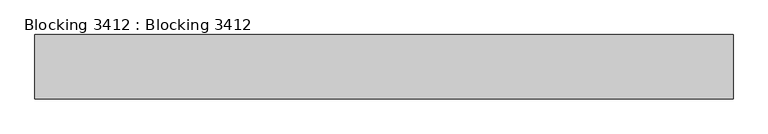
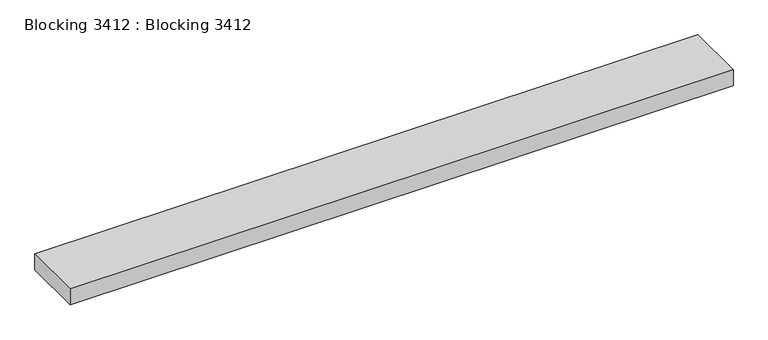
"""IFC4 building model written with IfcOpenShell, lengths in millimetres: proxy geometry, Blocking 3412 : Blocking 3412."""

from ifc_helpers import new_model, si_unit, frame, origin, place, context, project, spatial, polyline, outline, extrude, source, transform, mapped, element, save


def blocking_3412_blocking_3412_d82f70c8(model_context):
    return source(origin(), model_context, "Body", "SweptSolid", [
        extrude(outline(polyline([(3694.2883192, 10233.5061682), (3694.2883192, 10417.7250834), (5694.2883192, 10417.7250834), (5694.2883192, 10233.5061682), (3694.2883192, 10233.5061682)])), frame((0.0, 0.0, 39490.396), z_axis=(0.0, 0.0, 1.0), x_axis=(1.0, 0.0, 0.0)), (0.0, 0.0, 1.0), 50.8),
    ])


if __name__ == "__main__":
    model = new_model("IFC4")
    model_context = context("Model", 3, world=origin())
    ifc_project = project(units=[si_unit("LENGTHUNIT", "METRE", prefix="MILLI")], contexts=[model_context])
    site = spatial("IfcSite", under=ifc_project)
    building = spatial("IfcBuilding", under=site)
    placement = place(None, origin())
    blocking_3412_blocking_3412_shape = blocking_3412_blocking_3412_d82f70c8(model_context)
    element("IfcBuildingElementProxy", 1, Name="Blocking 3412 : Blocking 3412", ObjectType="Blocking 3412 : Blocking 3412", at=placement, inside=building, context=model_context, shape_type="MappedRepresentation", body=[
        mapped(blocking_3412_blocking_3412_shape, transform((0.0, 0.0, 0.0), x_axis=(1.0, 0.0, 0.0), y_axis=(0.0, 1.0, 0.0), z_axis=(0.0, 0.0, 1.0))),
    ])
    save(model, "model.ifc")

# Revit data of these elements
# Type "Blocking 3412 : Blocking 3412"
#   NameOverride = "Blocking"
# Element 1 (IfcBuildingElementProxy, "Blocking 3412 : Blocking 3412")
#   Materials on its faces: "WOOD BLOCKING AS REQUIRED"
# Materials
#   "WOOD BLOCKING AS REQUIRED": class "Unassigned", colour RGB 166 124 85, transparency 0, Cost = 0
